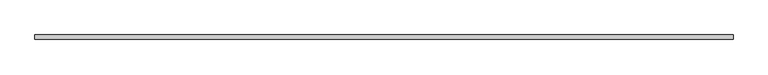
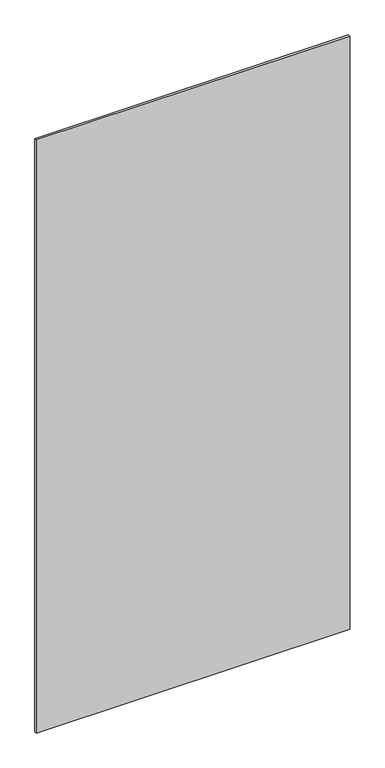
"""IFC4 building model written with IfcOpenShell, lengths in millimetres: proxy geometry, Panel:Panel:300402:Panel:300402 : Panel:Panel:300402:300124:Panel:300402:Panel:300402 : Panel:Panel:300402:300124 : Panel:Panel:300402:Panel:300402 : Panel:Panel:300402:300124:14 : Panel:Panel:300402:Panel:300402 : Panel:Panel:300402:300124:Panel:300402:Panel:300402 : Panel:Panel:300402:300124 : Panel:Panel:300402:Panel:300402 : Panel:Panel:300402:300124:300083."""

from ifc_helpers import new_model, si_unit, frame, origin, place, context, project, spatial, polyline, outline, extrude, source, transform, mapped, element, save


def generic_models_16cc9648(model_context):
    return source(origin(), model_context, "Body", "SweptSolid", [
        extrude(outline(polyline([(560648.2367239, -579076.8913841), (561867.4367239, -579076.8913841), (561867.4367239, -579084.8288841), (560648.2367239, -579084.8288841), (560648.2367239, -579076.8913841)])), frame((0.0, 0.0, 3695.7), z_axis=(0.0, 0.0, 1.0), x_axis=(1.0, 0.0, 0.0)), (0.0, 0.0, 1.0), 2438.4),
    ])


if __name__ == "__main__":
    model = new_model("IFC4")
    model_context = context("Model", 3, world=origin())
    ifc_project = project(units=[si_unit("LENGTHUNIT", "METRE", prefix="MILLI")], contexts=[model_context])
    site = spatial("IfcSite", under=ifc_project)
    building = spatial("IfcBuilding", under=site)
    placement = place(None, origin())
    generic_models_shape = generic_models_16cc9648(model_context)
    element("IfcBuildingElementProxy", 1, Name="Panel:Panel:300402:Panel:300402 : Panel:Panel:300402:300124:Panel:300402:Panel:300402 : Panel:Panel:300402:300124 : Panel:Panel:300402:Panel:300402 : Panel:Panel:300402:300124:14 : Panel:Panel:300402:Panel:300402 : Panel:Panel:300402:300124:Panel:300402:Panel:300402 : Panel:Panel:300402:300124 : Panel:Panel:300402:Panel:300402 : Panel:Panel:300402:300124:300083", ObjectType="Panel:Panel:300402:Panel:300402 : Panel:Panel:300402:300124:Panel:300402:Panel:300402 : Panel:Panel:300402:300124 : Panel:Panel:300402:Panel:300402 : Panel:Panel:300402:300124:14 : Panel:Panel:300402:Panel:300402 : Panel:Panel:300402:300124:Panel:300402:Panel:300402 : Panel:Panel:300402:300124 : Panel:Panel:300402:Panel:300402 : Panel:Panel:300402:300124:300083", at=placement, inside=building, context=model_context, shape_type="MappedRepresentation", body=[
        mapped(generic_models_shape, transform((0.0, 0.0, 0.0), x_axis=(1.0, 0.0, 0.0), y_axis=(0.0, 1.0, 0.0), z_axis=(0.0, 0.0, 1.0))),
    ])
    save(model, "model.ifc")

# Revit data of these elements
# Type "Panel:Panel:300402:Panel:300402 : Panel:Panel:300402:300124:Panel:300402:Panel:300402 : Panel:Panel:300402:300124 : Panel:Panel:300402:Panel:300402 : Panel:Panel:300402:300124:14 : Panel:Panel:300402:Panel:300402 : Panel:Panel:300402:300124:Panel:300402:Panel:300402 : Panel:Panel:300402:300124 : Panel:Panel:300402:Panel:300402 : Panel:Panel:300402:300124:300083"
#   NameOverride = "Panel:Panel:300402:Panel:300402 : Panel:Panel:300402:300124:Panel:300402:Panel:300402 : Panel:Panel:300402:300124 : Panel:Panel:300402:Panel:300402 : Panel:Panel:300402:300124:300083"
#   ObjectTypeOverride = "Panel:300402:Panel:300402 : Panel:Panel:300402:300124 : Panel:Panel:300402:Panel:300402 : Panel:Panel:300402:300124"
#   Reference = "Panel"
#   Tag = "300083"
# Element 1 (IfcBuildingElementProxy, "Panel:Panel:300402:Panel:300402 : Panel:Panel:300402:300124:Panel:300402:Panel:300402 : Panel:Panel:300402:300124 : Panel:Panel:300402:Panel:300402 : Panel:Panel:300402:300124:14 : Panel:Panel:300402:Panel:300402 : Panel:Panel:300402:300124:Panel:300402:Panel:300402 : Panel:Panel:300402:300124 : Panel:Panel:300402:Panel:300402 : Panel:Panel:300402:300124:300083")
#   Materials on its faces: "5/16\" PHENOLIC RESIN PANELS (CLASS A FLAME SPREAD) - EXPOSED FASTENERS"
# Materials
#   "5/16\" PHENOLIC RESIN PANELS (CLASS A FLAME SPREAD) - EXPOSED FASTENERS": class "Unassigned", colour RGB 64 64 64, transparency 0, Keynote = "M07420000.01", Cost = 0
